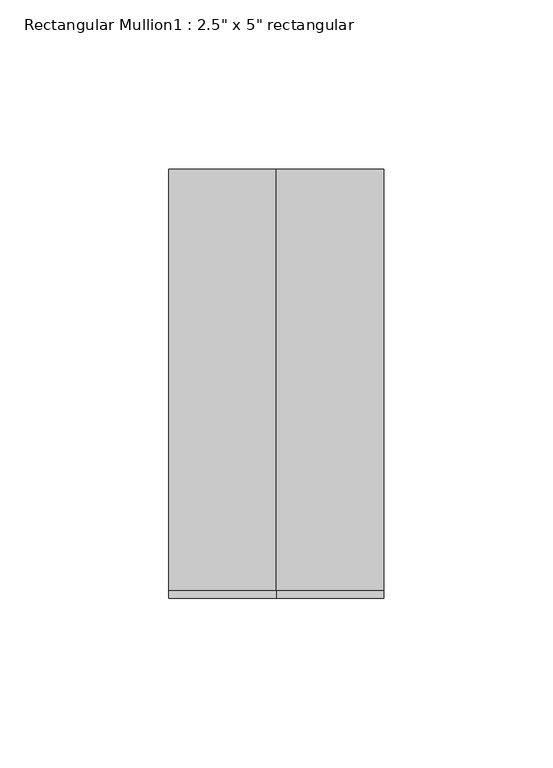
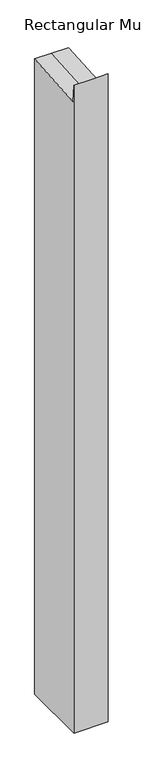
"""IFC4 building model written with IfcOpenShell, lengths in millimetres: member geometry."""

from ifc_helpers import new_model, si_unit, origin, place, context, project, spatial, faceted_brep, source, transform, mapped, element, save


def member_92e61aeb(model_context):
    return source(origin(), model_context, "Body", "Brep", [
        faceted_brep([(31.75, 63.5, -1249.2609667), (31.75, -63.5, -1249.2609667), (-31.75, -63.5, -1249.2609667), (-31.75, 63.5, -1249.2609667), (-31.75, 63.5, 4.3258089), (0.0, 63.5, 4.3258089), (31.75, 63.5, 4.3258089), (-31.75, -63.5, 29.5516342), (-31.75, -61.1522336, -4.315452), (31.75, -63.5, 29.5516342), (0.0, -63.5, 29.5516342), (31.75, -61.1522336, -4.315452), (0.0, -61.1522336, -4.315452)], [[[0, 1, 2, 3]], [[4, 5, 6, 0, 3]], [[7, 8, 4, 3, 2]], [[9, 10, 7, 2, 1]], [[6, 11, 9, 1, 0]], [[6, 5, 12, 11]], [[5, 4, 8, 12]], [[8, 7, 10, 12]], [[10, 9, 11, 12]]]),
    ])


if __name__ == "__main__":
    model = new_model("IFC4")
    model_context = context("Model", 3, world=origin())
    ifc_project = project(units=[si_unit("LENGTHUNIT", "METRE", prefix="MILLI")], contexts=[model_context])
    site = spatial("IfcSite", under=ifc_project)
    building = spatial("IfcBuilding", under=site)
    placement = place(None, origin())
    member_shape = member_92e61aeb(model_context)
    element("IfcMember", 1, ObjectType="Rectangular Mullion1 : 2.5\" x 5\" rectangular", at=placement, inside=building, context=model_context, shape_type="MappedRepresentation", body=[
        mapped(member_shape, transform((0.0, 0.0, 0.0), x_axis=(1.0, 0.0, 0.0), y_axis=(0.0, 1.0, 0.0), z_axis=(0.0, 0.0, 1.0))),
    ])
    save(model, "model.ifc")

# Revit data of these elements
# Type "Rectangular Mullion1 : 2.5\" x 5\" rectangular"
#   built-in parameter 1007304 = 0.416667 (stored number, unit not read)
#   built-in parameter 1007301 = 0.104167 (stored number, unit not read)
#   built-in parameter 1007300 = 0.104167 (stored number, unit not read)
# Element 1 (IfcMember, "Rectangular Mullion1 : 2.5\" x 5\" rectangular")
#   Materials on its faces: "support-frame"
# Materials
#   "support-frame": class "Unassigned", colour RGB 233 233 233, transparency 0, Cost = 0
